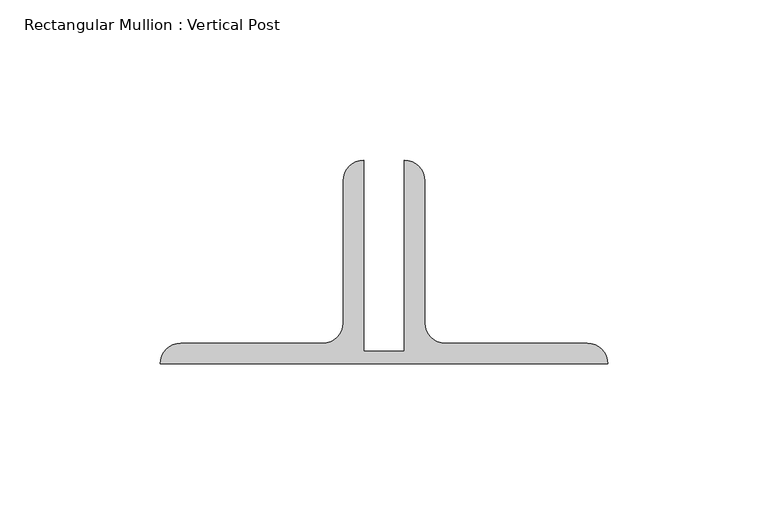
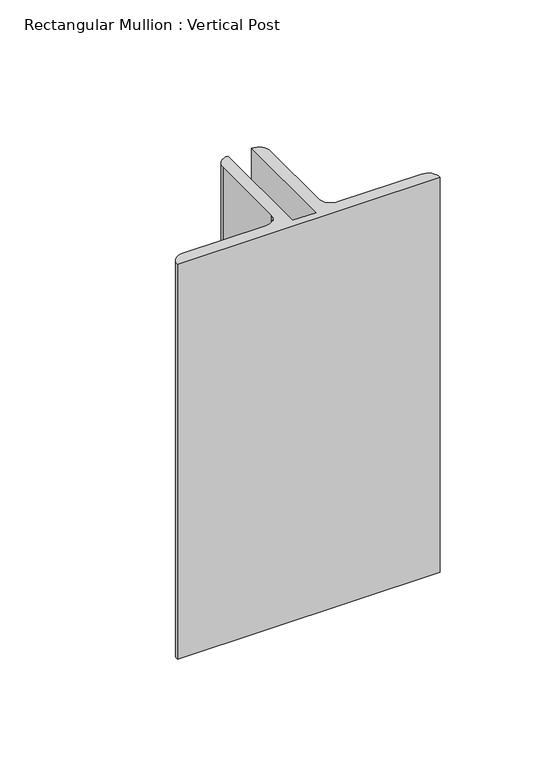
"""IFC4 building model written with IfcOpenShell, lengths in millimetres: member geometry, Rectangular Mullion : Vertical Post."""

import ifcopenshell
import ifcopenshell.guid

model = None  # the IFC model being written
_history = None  # IfcOwnerHistory: only IFC2X3 demands one
_inside = {}  # id of a spatial element -> (the spatial element, [elements in it])
_under = {}  # id of a project, library or spatial element -> (it, [spatial elements below it])
_declared = {}  # id of a project -> (the project, [libraries it declares])
_typed = {}  # id of a type object -> (the type object, [elements of that type])
_made_of = {}  # id of a material, layer set ... -> (it, [elements and type objects made of it])


def new_model(schema):
    """Start an empty IFC model of exactly this schema.

    Asked for "IFC4X3", IfcOpenShell would pick the latest addendum, in which some entities
    have other attributes; the version numbers below select the first issue.
    IFC2X3 requires an IfcOwnerHistory on every rooted entity: one is made here for all.
    """
    global model, _history
    if schema == "IFC4X3":
        model = ifcopenshell.file(schema_version=(4, 3, 0, 0))
    else:
        model = ifcopenshell.file(schema=schema)
    _inside.clear()
    _under.clear()
    _declared.clear()
    _typed.clear()
    _made_of.clear()
    _history = None
    if model.schema == "IFC2X3":
        org = make("IfcOrganization", Name="unknown")
        user = make(
            "IfcPersonAndOrganization",
            ThePerson=make("IfcPerson", FamilyName="unknown"),
            TheOrganization=org,
        )
        app = make(
            "IfcApplication",
            ApplicationDeveloper=org,
            Version="unknown",
            ApplicationFullName="unknown",
            ApplicationIdentifier="unknown",
        )
        _history = make(
            "IfcOwnerHistory",
            OwningUser=user,
            OwningApplication=app,
            ChangeAction="ADDED",
            CreationDate=0,
        )
    return model


def make(cls, **values):
    """One entity of the class cls with the attributes given. An attribute that is None is left unset."""
    return model.create_entity(
        cls, **{name: value for name, value in values.items() if value is not None}
    )


def rooted(cls, **values):
    """An entity with a GlobalId (a new one), such as an element, a storey or a relation."""
    return make(cls, GlobalId=ifcopenshell.guid.new(), OwnerHistory=_history, **values)


def si_unit(unit_type, name, prefix=None):
    """IfcSIUnit, for example si_unit("LENGTHUNIT", "METRE", prefix="MILLI")."""
    return make("IfcSIUnit", UnitType=unit_type, Prefix=prefix, Name=name)


def assignment(units):
    """IfcUnitAssignment: the units of a project."""
    return None if units is None else make("IfcUnitAssignment", Units=units)


def point(xyz):
    """IfcCartesianPoint."""
    return None if xyz is None else make("IfcCartesianPoint", Coordinates=xyz)


def direction(xyz):
    """IfcDirection."""
    return None if xyz is None else make("IfcDirection", DirectionRatios=xyz)


def frame(location, z_axis=None, x_axis=None):
    """IfcAxis2Placement3D, a coordinate frame: its origin and axes. An axis left out is left unset."""
    return make(
        "IfcAxis2Placement3D",
        Location=point(location),
        Axis=direction(z_axis),
        RefDirection=direction(x_axis),
    )


def frame_2d(location, x_axis=None):
    """IfcAxis2Placement2D, a coordinate frame in the plane: its origin and x axis."""
    return make(
        "IfcAxis2Placement2D", Location=point(location), RefDirection=direction(x_axis)
    )


def origin():
    """The frame at (0, 0, 0) with its axes left unset."""
    return frame((0.0, 0.0, 0.0))


def place(relative_to, where):
    """IfcLocalPlacement: puts the frame where relative to a parent placement (None: the world)."""
    return make(
        "IfcLocalPlacement", PlacementRelTo=relative_to, RelativePlacement=where
    )


def context(
    kind, dimensions, precision=None, world=None, true_north=None, identifier=None
):
    """IfcGeometricRepresentationContext, for example the 3D "Model" context."""
    return make(
        "IfcGeometricRepresentationContext",
        ContextIdentifier=identifier,
        ContextType=kind,
        CoordinateSpaceDimension=dimensions,
        Precision=precision,
        WorldCoordinateSystem=world,
        TrueNorth=true_north,
    )


def project(units=None, contexts=None):
    """IfcProject with its units and contexts."""
    return rooted(
        "IfcProject",
        Name="project",
        RepresentationContexts=contexts,
        UnitsInContext=assignment(units),
    )


def spatial(cls, under=None, at=None, **own):
    """A site, building, storey or space (cls), placed at a placement, below another one or the project."""
    s = rooted(cls, ObjectPlacement=at, **own)
    if under is not None:
        _under.setdefault(under.id(), (under, []))[1].append(s)
    return s


def polyline(points):
    """IfcPolyline through the points."""
    return make("IfcPolyline", Points=[point(p) for p in points])


def circle_curve(where, radius):
    """IfcCircle in the frame where."""
    return make("IfcCircle", Position=where, Radius=radius)


def trimmed(basis, trim1, trim2, sense, master):
    """IfcTrimmedCurve: the piece of a basis curve between two trims."""
    return make(
        "IfcTrimmedCurve",
        BasisCurve=basis,
        Trim1=trim1,
        Trim2=trim2,
        SenseAgreement=sense,
        MasterRepresentation=master,
    )


def segment(curve, same_sense, transition):
    """IfcCompositeCurveSegment."""
    return make(
        "IfcCompositeCurveSegment",
        Transition=transition,
        SameSense=same_sense,
        ParentCurve=curve,
    )


def composite_curve(segments, self_intersect=None):
    """IfcCompositeCurve: segments joined end to end."""
    return make("IfcCompositeCurve", Segments=segments, SelfIntersect=self_intersect)


def outline(outer, holes=None, kind="AREA"):
    """IfcArbitraryClosedProfileDef: a profile drawn as a closed curve; with holes, ...WithVoids."""
    if holes is None:
        return make("IfcArbitraryClosedProfileDef", ProfileType=kind, OuterCurve=outer)
    return make(
        "IfcArbitraryProfileDefWithVoids",
        ProfileType=kind,
        OuterCurve=outer,
        InnerCurves=holes,
    )


def extrude(swept, where, along, depth):
    """IfcExtrudedAreaSolid: the profile swept, set in the frame where, extruded along a direction by depth."""
    return make(
        "IfcExtrudedAreaSolid",
        SweptArea=swept,
        Position=where,
        ExtrudedDirection=direction(along),
        Depth=depth,
    )


def shape(context_of_items, identifier, shape_type, items):
    """IfcShapeRepresentation: the items that make up one representation, for example the "Body"."""
    return make(
        "IfcShapeRepresentation",
        ContextOfItems=context_of_items,
        RepresentationIdentifier=identifier,
        RepresentationType=shape_type,
        Items=items,
    )


def source(mapping_origin, context_of_items, identifier, shape_type, items):
    """IfcRepresentationMap: a shape defined once, which mapped items show again and again."""
    return make(
        "IfcRepresentationMap",
        MappingOrigin=mapping_origin,
        MappedRepresentation=shape(context_of_items, identifier, shape_type, items),
    )


def transform(
    local_origin,
    x_axis=None,
    y_axis=None,
    z_axis=None,
    scale=None,
    scale2=None,
    scale3=None,
    uniform=True,
):
    """IfcCartesianTransformationOperator3D, or its non-uniform kind. x_axis, y_axis, z_axis: its Axis1, 2, 3."""
    if uniform:
        return make(
            "IfcCartesianTransformationOperator3D",
            Axis1=direction(x_axis),
            Axis2=direction(y_axis),
            LocalOrigin=point(local_origin),
            Scale=scale,
            Axis3=direction(z_axis),
        )
    return make(
        "IfcCartesianTransformationOperator3DnonUniform",
        Axis1=direction(x_axis),
        Axis2=direction(y_axis),
        LocalOrigin=point(local_origin),
        Scale=scale,
        Axis3=direction(z_axis),
        Scale2=scale2,
        Scale3=scale3,
    )


def mapped(mapping_source, mapping_target):
    """IfcMappedItem: shows the shape of a source again, moved by a transform."""
    return make(
        "IfcMappedItem", MappingSource=mapping_source, MappingTarget=mapping_target
    )


def made_of(thing, what):
    """Note that an element or type object is made of a material, layer set ...; save() writes the relation."""
    if what is not None:
        _made_of.setdefault(what.id(), (what, []))[1].append(thing)
    return thing


def element(
    cls,
    number,
    at=None,
    inside=None,
    cuts=None,
    type_object=None,
    material=None,
    context=None,
    identifier="Body",
    shape_type=None,
    held_by="IfcProductDefinitionShape",
    body=None,
    shapes=None,
    **own,
):
    """One element of the class cls, such as IfcWall. Its Tag is "e" and its number.

    at: its placement. inside: the storey or other place that contains it. cuts: it is an
    opening in that element (IfcRelVoidsElement). A single representation is given by context,
    identifier, shape_type and body (its items); several are given by shapes. held_by: the class
    of the entity that holds the representations. save() writes the other relations.
    """
    e = rooted(cls, Tag="e%d" % number, ObjectPlacement=at, **own)
    if body is not None:
        shapes = [shape(context, identifier, shape_type, body)]
    if shapes is not None:
        e.Representation = make(held_by, Representations=shapes)
    if inside is not None:
        _inside.setdefault(inside.id(), (inside, []))[1].append(e)
    if cuts is not None:
        rooted(
            "IfcRelVoidsElement", RelatingBuildingElement=cuts, RelatedOpeningElement=e
        )
    if type_object is not None:
        _typed.setdefault(type_object.id(), (type_object, []))[1].append(e)
    return made_of(e, material)


def aggregate(whole, parts):
    """IfcRelAggregates: a whole, such as a stair, and the parts it consists of."""
    return rooted("IfcRelAggregates", RelatingObject=whole, RelatedObjects=parts)


def save(model, path):
    """Write the relations noted so far, then the file.

    IfcRelAggregates (storeys below a building ...), IfcRelContainedInSpatialStructure (elements
    in a storey), IfcRelDefinesByType, IfcRelAssociatesMaterial and IfcRelDeclares: one each for
    every whole, place, type object, material and project.
    """
    for whole, parts in _under.values():
        aggregate(whole, parts)
    for where, things in _inside.values():
        rooted(
            "IfcRelContainedInSpatialStructure",
            RelatedElements=things,
            RelatingStructure=where,
        )
    for kind, things in _typed.values():
        rooted("IfcRelDefinesByType", RelatedObjects=things, RelatingType=kind)
    for what, things in _made_of.values():
        rooted("IfcRelAssociatesMaterial", RelatedObjects=things, RelatingMaterial=what)
    for by, libraries in _declared.values():
        rooted("IfcRelDeclares", RelatingContext=by, RelatedDefinitions=libraries)
    model.write(path)


def rectangular_mullion_vertical_post_d81d6a22(model_context):
    return source(origin(), model_context, "Body", "SweptSolid", [
        extrude(outline(composite_curve([segment(polyline([(-6.35, 22.9145205), (6.35, 22.9145205), (6.35, 82.55)]), True, "CONTINUOUS"), segment(trimmed(circle_curve(frame_2d((6.35, 76.2)), 6.35), [point((6.35, 82.55))], [point((12.7, 76.2))], False, "CARTESIAN"), True, "CONTINUOUS"), segment(polyline([(12.7, 76.2), (12.7, 31.75)]), True, "CONTINUOUS"), segment(trimmed(circle_curve(frame_2d((19.05, 31.75)), 6.35), [point((12.7, 31.75))], [point((19.05, 25.4))], True, "CARTESIAN"), True, "CONTINUOUS"), segment(polyline([(19.05, 25.4), (63.5, 25.4)]), True, "CONTINUOUS"), segment(trimmed(circle_curve(frame_2d((63.5, 19.05)), 6.35), [point((63.5, 25.4))], [point((69.85, 19.05))], False, "CARTESIAN"), True, "CONTINUOUS"), segment(polyline([(69.85, 19.05), (-69.85, 19.05)]), True, "CONTINUOUS"), segment(trimmed(circle_curve(frame_2d((-63.5, 19.05)), 6.35), [point((-69.85, 19.05))], [point((-63.5, 25.4))], False, "CARTESIAN"), True, "CONTINUOUS"), segment(polyline([(-63.5, 25.4), (-19.05, 25.4)]), True, "CONTINUOUS"), segment(trimmed(circle_curve(frame_2d((-19.05, 31.75)), 6.35), [point((-19.05, 25.4))], [point((-12.7, 31.75))], True, "CARTESIAN"), True, "CONTINUOUS"), segment(polyline([(-12.7, 31.75), (-12.7, 76.2)]), True, "CONTINUOUS"), segment(trimmed(circle_curve(frame_2d((-6.35, 76.2)), 6.35), [point((-12.7, 76.2))], [point((-6.35, 82.55))], False, "CARTESIAN"), True, "CONTINUOUS"), segment(polyline([(-6.35, 82.55), (-6.35, 22.9145205)]), True, "CONTINUOUS")], self_intersect=False)), frame((0.0, 0.0, -222.0889998), z_axis=(0.0, 0.0, 1.0), x_axis=(1.0, 0.0, 0.0)), (0.0, 0.0, 1.0), 222.0889998),
    ])


if __name__ == "__main__":
    model = new_model("IFC4")
    model_context = context("Model", 3, world=origin())
    ifc_project = project(units=[si_unit("LENGTHUNIT", "METRE", prefix="MILLI")], contexts=[model_context])
    site = spatial("IfcSite", under=ifc_project)
    building = spatial("IfcBuilding", under=site)
    placement = place(None, origin())
    rectangular_mullion_vertical_post_shape = rectangular_mullion_vertical_post_d81d6a22(model_context)
    element("IfcMember", 1, ObjectType="Rectangular Mullion : Vertical Post", at=placement, inside=building, context=model_context, shape_type="MappedRepresentation", body=[
        mapped(rectangular_mullion_vertical_post_shape, transform((0.0, 0.0, 0.0), x_axis=(1.0, 0.0, 0.0), y_axis=(0.0, 1.0, 0.0), z_axis=(0.0, 0.0, 1.0))),
    ])
    save(model, "model.ifc")

# Revit data of these elements
# Type "Rectangular Mullion : Vertical Post"
#   built-in parameter 1007351 = -0.0625 (stored number, unit not read)
#   built-in parameter 1007322 = 0.0126789 (stored number, unit not read)
#   built-in parameter 1007321 = 0.229167 (stored number, unit not read)
#   built-in parameter 1007320 = 0.229167 (stored number, unit not read)
# Element 1 (IfcMember, "Rectangular Mullion : Vertical Post")
#   Materials on its faces: "GATE POST: GALVANIZED ANGLES"
# Materials
#   "GATE POST: GALVANIZED ANGLES": class "Unassigned", colour RGB 211 211 211, transparency 0, Cost = 0
